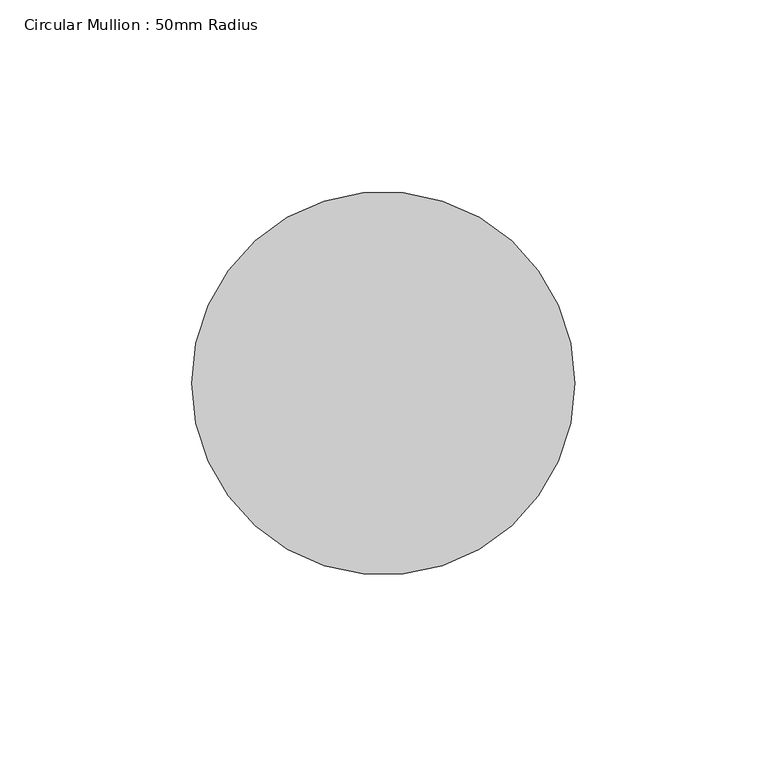
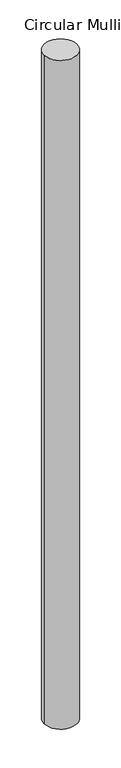
"""IFC4 building model written with IfcOpenShell, lengths in millimetres: member geometry, Circular Mullion : 50mm Radius."""

from ifc_helpers import new_model, si_unit, point, frame, origin, origin_2d, place, context, project, spatial, circle_curve, trimmed, segment, composite_curve, outline, extrude, source, transform, mapped, element, save


def circular_mullion_50mm_radius_40c9dc8a(model_context):
    return source(origin(), model_context, "Body", "SweptSolid", [
        extrude(outline(composite_curve([segment(trimmed(circle_curve(origin_2d(), 50.0), [point((50.0, 0.0))], [point((-50.0, 0.0))], False, "CARTESIAN"), True, "CONTINUOUS"), segment(trimmed(circle_curve(origin_2d(), 50.0), [point((-50.0, 0.0))], [point((50.0, 0.0))], False, "CARTESIAN"), True, "CONTINUOUS")], self_intersect=False)), frame((0.0, 0.0, -2157.8661597), z_axis=(0.0, 0.0, 1.0), x_axis=(1.0, 0.0, 0.0)), (0.0, 0.0, 1.0), 2157.8661597),
    ])


if __name__ == "__main__":
    model = new_model("IFC4")
    model_context = context("Model", 3, world=origin())
    ifc_project = project(units=[si_unit("LENGTHUNIT", "METRE", prefix="MILLI")], contexts=[model_context])
    site = spatial("IfcSite", under=ifc_project)
    building = spatial("IfcBuilding", under=site)
    placement = place(None, origin())
    circular_mullion_50mm_radius_shape = circular_mullion_50mm_radius_40c9dc8a(model_context)
    element("IfcMember", 1, ObjectType="Circular Mullion : 50mm Radius", at=placement, inside=building, context=model_context, shape_type="MappedRepresentation", body=[
        mapped(circular_mullion_50mm_radius_shape, transform((0.0, 0.0, 0.0), x_axis=(1.0, 0.0, 0.0), y_axis=(0.0, 1.0, 0.0), z_axis=(0.0, 0.0, 1.0))),
    ])
    save(model, "model.ifc")

# Revit data of these elements
# Type "Circular Mullion : 50mm Radius"
#   built-in parameter 1007350 = 0.164042 (stored number, unit not read)
# Element 1 (IfcMember, "Circular Mullion : 50mm Radius")
#   Materials on its faces: "Aluminium"
# Materials
#   "Aluminium": class "Metal", colour RGB 247 247 247, transparency 0, Description = "Aluminium 6061", Cost = 0
